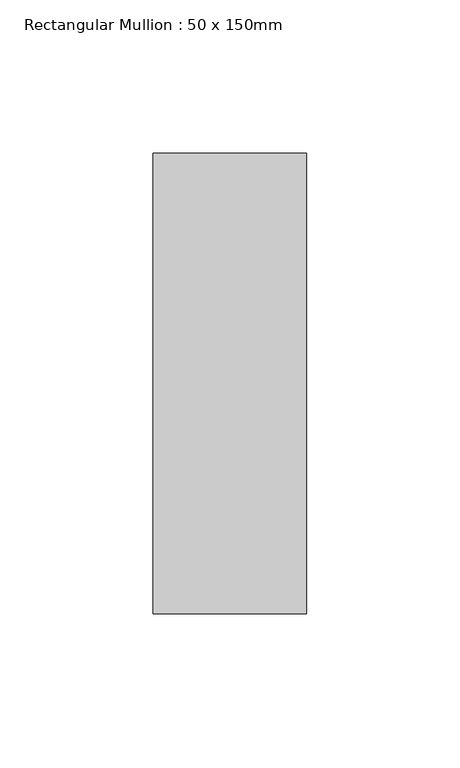
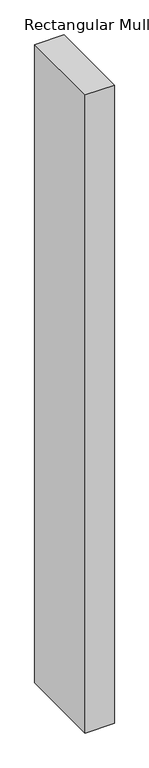
"""IFC4 building model written with IfcOpenShell, lengths in millimetres: member geometry, Rectangular Mullion : 50 x 150mm."""

from ifc_helpers import new_model, si_unit, frame, origin, place, context, project, spatial, polyline, outline, extrude, source, transform, mapped, element, save


def rectangular_mullion_50_x_150mm_1f9b408c(model_context):
    return source(origin(), model_context, "Body", "SweptSolid", [
        extrude(outline(polyline([(0.0, 75.0), (0.0, -75.0), (-50.0, -75.0), (-50.0, 75.0), (0.0, 75.0)])), frame((0.0, 0.0, -1158.3333333), z_axis=(0.0, 0.0, 1.0), x_axis=(1.0, 0.0, 0.0)), (0.0, 0.0, 1.0), 1158.3333333),
    ])


if __name__ == "__main__":
    model = new_model("IFC4")
    model_context = context("Model", 3, world=origin())
    ifc_project = project(units=[si_unit("LENGTHUNIT", "METRE", prefix="MILLI")], contexts=[model_context])
    site = spatial("IfcSite", under=ifc_project)
    building = spatial("IfcBuilding", under=site)
    placement = place(None, origin())
    rectangular_mullion_50_x_150mm_shape = rectangular_mullion_50_x_150mm_1f9b408c(model_context)
    element("IfcMember", 1, ObjectType="Rectangular Mullion : 50 x 150mm", at=placement, inside=building, context=model_context, shape_type="MappedRepresentation", body=[
        mapped(rectangular_mullion_50_x_150mm_shape, transform((0.0, 0.0, 0.0), x_axis=(1.0, 0.0, 0.0), y_axis=(0.0, 1.0, 0.0), z_axis=(0.0, 0.0, 1.0))),
    ])
    save(model, "model.ifc")

# Revit data of these elements
# Type "Rectangular Mullion : 50 x 150mm"
#   built-in parameter 1007304 = 0.492126 (stored number, unit not read)
#   built-in parameter 1007301 = 0.082021 (stored number, unit not read)
#   built-in parameter 1007300 = 0.082021 (stored number, unit not read)
# Element 1 (IfcMember, "Rectangular Mullion : 50 x 150mm")
#   Materials on its faces: "Metal - Aluminium"
# Materials
#   "Metal - Aluminium": class "Metal", colour RGB 247 247 247, transparency 0
